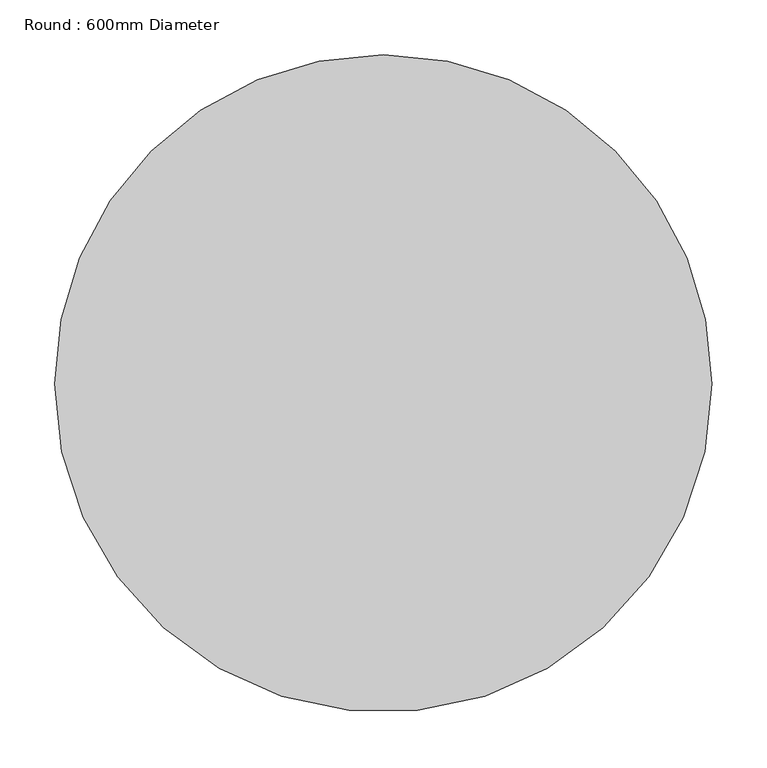
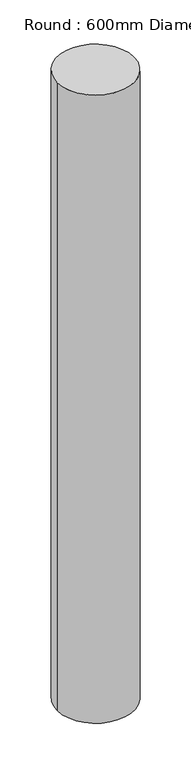
"""IFC4 building model written with IfcOpenShell, lengths in millimetres: column geometry, Round : 600mm Diameter."""

from ifc_helpers import new_model, si_unit, point, frame, origin, origin_2d, place, context, project, spatial, circle_curve, trimmed, segment, composite_curve, outline, extrude, source, transform, mapped, element, save


def round_600mm_diameter_42bc9892(model_context):
    return source(origin(), model_context, "Body", "SweptSolid", [
        extrude(outline(composite_curve([segment(trimmed(circle_curve(origin_2d(), 300.0), [point((300.0, 0.0))], [point((-300.0, 0.0))], False, "CARTESIAN"), True, "CONTINUOUS"), segment(trimmed(circle_curve(origin_2d(), 300.0), [point((-300.0, 0.0))], [point((0.0, 300.0))], False, "CARTESIAN"), True, "CONTINUOUS"), segment(trimmed(circle_curve(origin_2d(), 300.0), [point((0.0, 300.0))], [point((300.0, 0.0))], False, "CARTESIAN"), True, "CONTINUOUS")], self_intersect=False)), frame((0.0, 0.0, 125100.0), z_axis=(0.0, 0.0, 1.0), x_axis=(1.0, 0.0, 0.0)), (0.0, 0.0, 1.0), 5170.0),
    ])


if __name__ == "__main__":
    model = new_model("IFC4")
    model_context = context("Model", 3, world=origin())
    ifc_project = project(units=[si_unit("LENGTHUNIT", "METRE", prefix="MILLI")], contexts=[model_context])
    site = spatial("IfcSite", under=ifc_project)
    building = spatial("IfcBuilding", under=site)
    placement = place(None, origin())
    round_600mm_diameter_shape = round_600mm_diameter_42bc9892(model_context)
    element("IfcColumn", 1, ObjectType="Round : 600mm Diameter", at=placement, inside=building, context=model_context, shape_type="MappedRepresentation", body=[
        mapped(round_600mm_diameter_shape, transform((0.0, 0.0, 0.0), x_axis=(1.0, 0.0, 0.0), y_axis=(0.0, 1.0, 0.0), z_axis=(0.0, 0.0, 1.0))),
    ])
    save(model, "model.ifc")

# Revit data of these elements
# Type "Round : 600mm Diameter"
#   Keynote = "G"
#   Diameter = 600.00 mm
#   Offset Base = 0.00 mm
#   Offset Top = 0.00 mm
#   built-in parameter 1002110 = 8421504
#   built-in parameter 1002106 = element 3
#   Material = Concrete - Cast In Situ
# Element 1 (IfcColumn, "Round : 600mm Diameter")
#   Materials on its faces: "Concrete - Cast In Situ"
# Materials
#   "Concrete - Cast In Situ": class "Unassigned", colour RGB 255 255 255, transparency 0, Keynote = "E10/132", Cost = 0
